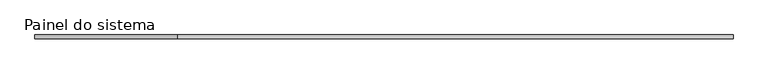
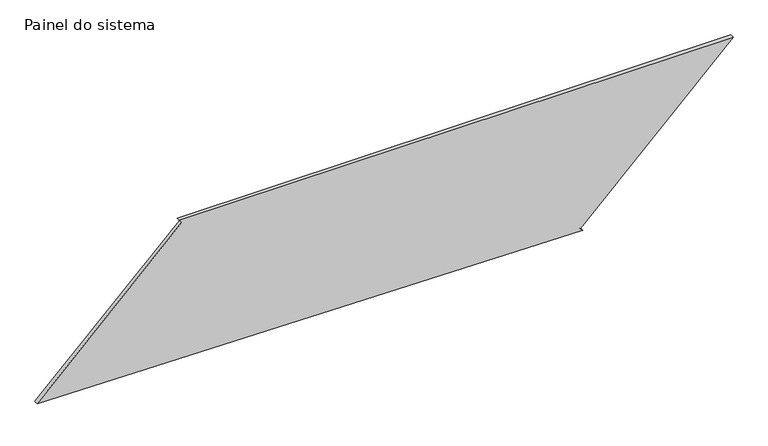
"""IFC4 building model written with IfcOpenShell, lengths in millimetres: plate geometry, Painel do sistema : Envidraçado."""

from ifc_helpers import new_model, si_unit, frame, origin, place, context, project, spatial, polyline, outline, extrude, source, transform, mapped, element, save


def painel_do_sistema_bdc7579c(model_context):
    return source(origin(), model_context, "Body", "SweptSolid", [
        extrude(outline(polyline([(0.0, 1304.0794831), (17.9061609, 1286.6332973), (999.2894187, 2293.8910849), (999.2894187, -1356.8050629), (981.3832578, -1339.3588771), (51.3711603, -2293.8910849), (0.0, 1304.0794831)])), frame((0.0, 24.5, 0.0), z_axis=(0.0, 1.0, 0.0), x_axis=(0.0, 0.0, 1.0)), (0.0, 0.0, 1.0), 25.0),
    ])


if __name__ == "__main__":
    model = new_model("IFC4")
    model_context = context("Model", 3, world=origin())
    ifc_project = project(units=[si_unit("LENGTHUNIT", "METRE", prefix="MILLI")], contexts=[model_context])
    site = spatial("IfcSite", under=ifc_project)
    building = spatial("IfcBuilding", under=site)
    placement = place(None, origin())
    painel_do_sistema_shape = painel_do_sistema_bdc7579c(model_context)
    element("IfcPlate", 1, ObjectType="Painel do sistema : Envidraçado", at=placement, inside=building, context=model_context, shape_type="MappedRepresentation", body=[
        mapped(painel_do_sistema_shape, transform((0.0, 0.0, 0.0), x_axis=(1.0, 0.0, 0.0), y_axis=(0.0, 1.0, 0.0), z_axis=(0.0, 0.0, 1.0))),
    ])
    save(model, "model.ifc")

# Revit data of these elements
# Type "Painel do sistema : Envidraçado"
#   Construction Type Id = "GSP4R"
#   Analytic Construction = "Vidraça única Pilkington 1/8 pol"
#   Visual Light Transmittance = 0.9
#   Solar Heat Gain Coefficient = 0.86
#   Heat Transfer Coefficient (U) = 6.7069 W/(m²·K)
# Element 1 (IfcPlate, "Painel do sistema : Envidraçado")
#   Materials on its faces: "Vidro"
# Materials
#   "Vidro": class "Vidro", colour RGB 0 128 192, transparency 0.9, Description = "Vidro de sílica", Cost = 0
